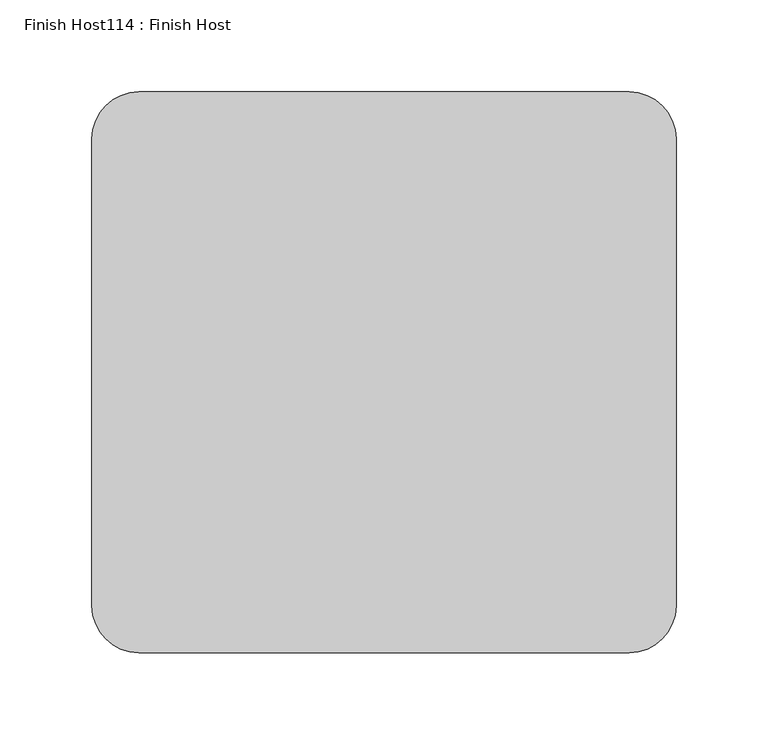
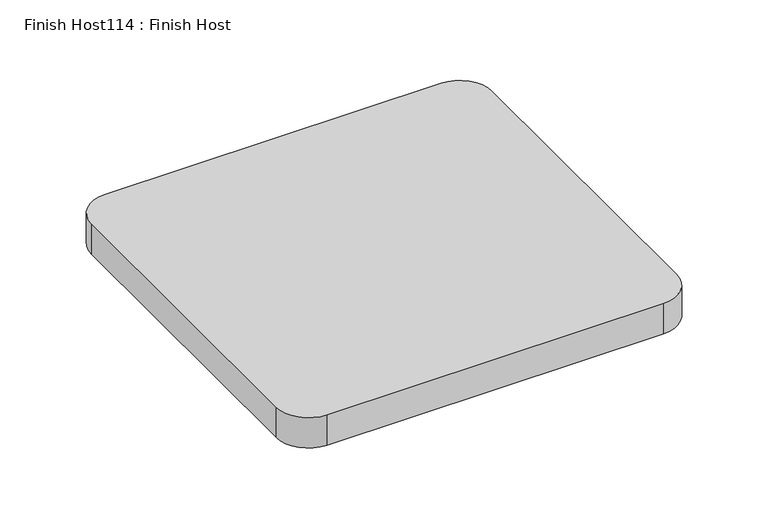
"""IFC4 building model written with IfcOpenShell, lengths in millimetres: proxy geometry, Finish Host114 : Finish Host."""

from ifc_helpers import new_model, si_unit, point, frame_2d, origin, origin_with_axes, place, context, project, spatial, polyline, circle_curve, trimmed, segment, composite_curve, outline, extrude, source, transform, mapped, element, save


def finish_host114_finish_host_c530d4e4(model_context):
    return source(origin(), model_context, "Body", "SweptSolid", [
        extrude(outline(composite_curve([segment(polyline([(-797.1842816, 3462.3960864), (-797.1842816, 3716.3960864)]), True, "CONTINUOUS"), segment(trimmed(circle_curve(frame_2d((-771.7842816, 3716.3960864)), 25.4), [point((-797.1842816, 3716.3960864))], [point((-771.7842816, 3741.7960864))], False, "CARTESIAN"), True, "CONTINUOUS"), segment(polyline([(-771.7842816, 3741.7960864), (-505.0842816, 3741.7960864)]), True, "CONTINUOUS"), segment(trimmed(circle_curve(frame_2d((-505.0842816, 3716.3960864)), 25.4), [point((-505.0842816, 3741.7960864))], [point((-479.6842816, 3716.3960864))], False, "CARTESIAN"), True, "CONTINUOUS"), segment(polyline([(-479.6842816, 3716.3960864), (-479.6842816, 3462.3960864)]), True, "CONTINUOUS"), segment(trimmed(circle_curve(frame_2d((-505.0842816, 3462.3960864)), 25.4), [point((-479.6842816, 3462.3960864))], [point((-505.0842816, 3436.9960864))], False, "CARTESIAN"), True, "CONTINUOUS"), segment(polyline([(-505.0842816, 3436.9960864), (-771.7842816, 3436.9960864)]), True, "CONTINUOUS"), segment(trimmed(circle_curve(frame_2d((-771.7842816, 3462.3960864)), 25.4), [point((-771.7842816, 3436.9960864))], [point((-797.1842816, 3462.3960864))], False, "CARTESIAN"), True, "CONTINUOUS")], self_intersect=False)), origin_with_axes(), (0.0, 0.0, 1.0), 25.4),
    ])


if __name__ == "__main__":
    model = new_model("IFC4")
    model_context = context("Model", 3, world=origin())
    ifc_project = project(units=[si_unit("LENGTHUNIT", "METRE", prefix="MILLI")], contexts=[model_context])
    site = spatial("IfcSite", under=ifc_project)
    building = spatial("IfcBuilding", under=site)
    placement = place(None, origin())
    finish_host114_finish_host_shape = finish_host114_finish_host_c530d4e4(model_context)
    element("IfcBuildingElementProxy", 1, Name="Finish Host114 : Finish Host", ObjectType="Finish Host114 : Finish Host", at=placement, inside=building, context=model_context, shape_type="MappedRepresentation", body=[
        mapped(finish_host114_finish_host_shape, transform((0.0, 0.0, 0.0), x_axis=(1.0, 0.0, 0.0), y_axis=(0.0, 1.0, 0.0), z_axis=(0.0, 0.0, 1.0))),
    ])
    save(model, "model.ifc")

# Revit data of these elements
# Type "Finish Host114 : Finish Host"
#   Panel Material = Fabric - Teknion - M213 - Meme - Buzz
# Element 1 (IfcBuildingElementProxy, "Finish Host114 : Finish Host")
#   Materials on its faces: "Fabric - Teknion - M213 - Meme - Buzz"
# Materials
#   "Fabric - Teknion - M213 - Meme - Buzz": class "Fabric", colour RGB 57 57 55, transparency 0, Model = "M213", Manufacturer = "Teknion Studios", URL = "http://www.teknionstudio.com/", Description = "Buzz Meme", Cost = 0
